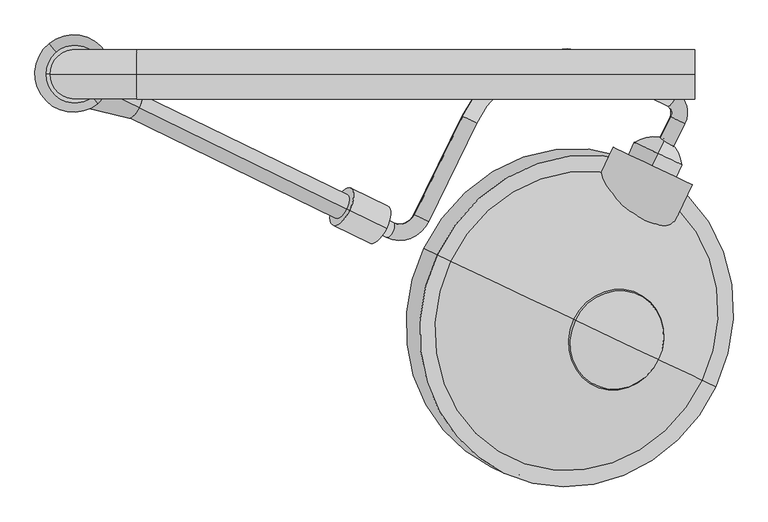
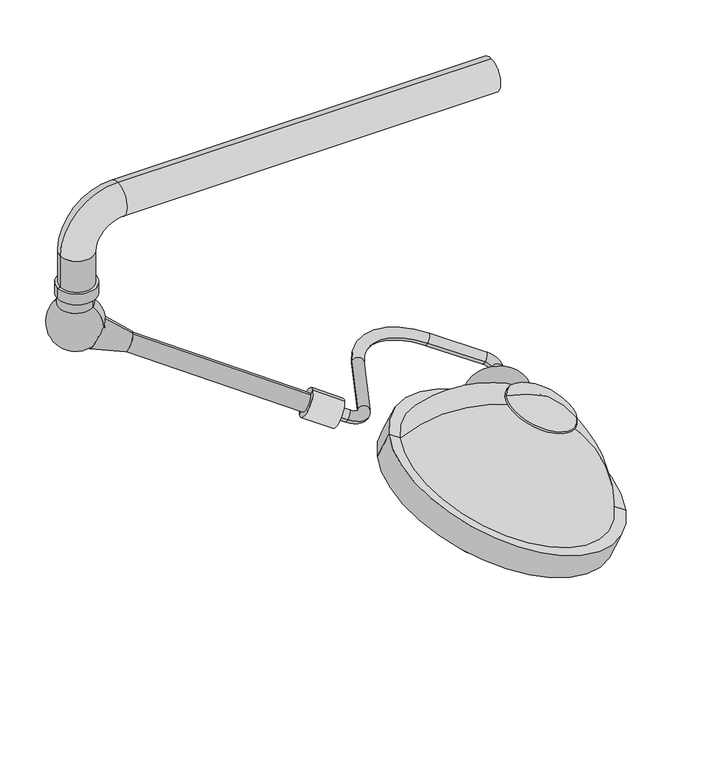
"""IFC4 building model written with IfcOpenShell, lengths in millimetres: proxy geometry, M7490 - Light, Surg, Ceiling Mtd, Dual, Unequal Dia Heads : M7490 - Light, Surg, Ceiling Mtd, Dual, Unequal Dia Heads."""

import ifcopenshell
import ifcopenshell.guid

model = None  # the IFC model being written
_history = None  # IfcOwnerHistory: only IFC2X3 demands one
_inside = {}  # id of a spatial element -> (the spatial element, [elements in it])
_under = {}  # id of a project, library or spatial element -> (it, [spatial elements below it])
_declared = {}  # id of a project -> (the project, [libraries it declares])
_typed = {}  # id of a type object -> (the type object, [elements of that type])
_made_of = {}  # id of a material, layer set ... -> (it, [elements and type objects made of it])


def new_model(schema):
    """Start an empty IFC model of exactly this schema.

    Asked for "IFC4X3", IfcOpenShell would pick the latest addendum, in which some entities
    have other attributes; the version numbers below select the first issue.
    IFC2X3 requires an IfcOwnerHistory on every rooted entity: one is made here for all.
    """
    global model, _history
    if schema == "IFC4X3":
        model = ifcopenshell.file(schema_version=(4, 3, 0, 0))
    else:
        model = ifcopenshell.file(schema=schema)
    _inside.clear()
    _under.clear()
    _declared.clear()
    _typed.clear()
    _made_of.clear()
    _history = None
    if model.schema == "IFC2X3":
        org = make("IfcOrganization", Name="unknown")
        user = make(
            "IfcPersonAndOrganization",
            ThePerson=make("IfcPerson", FamilyName="unknown"),
            TheOrganization=org,
        )
        app = make(
            "IfcApplication",
            ApplicationDeveloper=org,
            Version="unknown",
            ApplicationFullName="unknown",
            ApplicationIdentifier="unknown",
        )
        _history = make(
            "IfcOwnerHistory",
            OwningUser=user,
            OwningApplication=app,
            ChangeAction="ADDED",
            CreationDate=0,
        )
    return model


def make(cls, **values):
    """One entity of the class cls with the attributes given. An attribute that is None is left unset."""
    return model.create_entity(
        cls, **{name: value for name, value in values.items() if value is not None}
    )


def rooted(cls, **values):
    """An entity with a GlobalId (a new one), such as an element, a storey or a relation."""
    return make(cls, GlobalId=ifcopenshell.guid.new(), OwnerHistory=_history, **values)


def si_unit(unit_type, name, prefix=None):
    """IfcSIUnit, for example si_unit("LENGTHUNIT", "METRE", prefix="MILLI")."""
    return make("IfcSIUnit", UnitType=unit_type, Prefix=prefix, Name=name)


def assignment(units):
    """IfcUnitAssignment: the units of a project."""
    return None if units is None else make("IfcUnitAssignment", Units=units)


def point(xyz):
    """IfcCartesianPoint."""
    return None if xyz is None else make("IfcCartesianPoint", Coordinates=xyz)


def direction(xyz):
    """IfcDirection."""
    return None if xyz is None else make("IfcDirection", DirectionRatios=xyz)


def frame(location, z_axis=None, x_axis=None):
    """IfcAxis2Placement3D, a coordinate frame: its origin and axes. An axis left out is left unset."""
    return make(
        "IfcAxis2Placement3D",
        Location=point(location),
        Axis=direction(z_axis),
        RefDirection=direction(x_axis),
    )


def frame_2d(location, x_axis=None):
    """IfcAxis2Placement2D, a coordinate frame in the plane: its origin and x axis."""
    return make(
        "IfcAxis2Placement2D", Location=point(location), RefDirection=direction(x_axis)
    )


def origin():
    """The frame at (0, 0, 0) with its axes left unset."""
    return frame((0.0, 0.0, 0.0))


def origin_2d():
    """The frame at (0, 0) in the plane with its x axis left unset."""
    return frame_2d((0.0, 0.0))


def place(relative_to, where):
    """IfcLocalPlacement: puts the frame where relative to a parent placement (None: the world)."""
    return make(
        "IfcLocalPlacement", PlacementRelTo=relative_to, RelativePlacement=where
    )


def context(
    kind, dimensions, precision=None, world=None, true_north=None, identifier=None
):
    """IfcGeometricRepresentationContext, for example the 3D "Model" context."""
    return make(
        "IfcGeometricRepresentationContext",
        ContextIdentifier=identifier,
        ContextType=kind,
        CoordinateSpaceDimension=dimensions,
        Precision=precision,
        WorldCoordinateSystem=world,
        TrueNorth=true_north,
    )


def project(units=None, contexts=None):
    """IfcProject with its units and contexts."""
    return rooted(
        "IfcProject",
        Name="project",
        RepresentationContexts=contexts,
        UnitsInContext=assignment(units),
    )


def spatial(cls, under=None, at=None, **own):
    """A site, building, storey or space (cls), placed at a placement, below another one or the project."""
    s = rooted(cls, ObjectPlacement=at, **own)
    if under is not None:
        _under.setdefault(under.id(), (under, []))[1].append(s)
    return s


def polyline(points):
    """IfcPolyline through the points."""
    return make("IfcPolyline", Points=[point(p) for p in points])


def circle_curve(where, radius):
    """IfcCircle in the frame where."""
    return make("IfcCircle", Position=where, Radius=radius)


def ellipse_curve(where, semi_axis1, semi_axis2):
    """IfcEllipse in the frame where."""
    return make(
        "IfcEllipse", Position=where, SemiAxis1=semi_axis1, SemiAxis2=semi_axis2
    )


def trimmed(basis, trim1, trim2, sense, master):
    """IfcTrimmedCurve: the piece of a basis curve between two trims."""
    return make(
        "IfcTrimmedCurve",
        BasisCurve=basis,
        Trim1=trim1,
        Trim2=trim2,
        SenseAgreement=sense,
        MasterRepresentation=master,
    )


def segment(curve, same_sense, transition):
    """IfcCompositeCurveSegment."""
    return make(
        "IfcCompositeCurveSegment",
        Transition=transition,
        SameSense=same_sense,
        ParentCurve=curve,
    )


def composite_curve(segments, self_intersect=None):
    """IfcCompositeCurve: segments joined end to end."""
    return make("IfcCompositeCurve", Segments=segments, SelfIntersect=self_intersect)


def outline(outer, holes=None, kind="AREA"):
    """IfcArbitraryClosedProfileDef: a profile drawn as a closed curve; with holes, ...WithVoids."""
    if holes is None:
        return make("IfcArbitraryClosedProfileDef", ProfileType=kind, OuterCurve=outer)
    return make(
        "IfcArbitraryProfileDefWithVoids",
        ProfileType=kind,
        OuterCurve=outer,
        InnerCurves=holes,
    )


def extrude(swept, where, along, depth):
    """IfcExtrudedAreaSolid: the profile swept, set in the frame where, extruded along a direction by depth."""
    return make(
        "IfcExtrudedAreaSolid",
        SweptArea=swept,
        Position=where,
        ExtrudedDirection=direction(along),
        Depth=depth,
    )


def shape(context_of_items, identifier, shape_type, items):
    """IfcShapeRepresentation: the items that make up one representation, for example the "Body"."""
    return make(
        "IfcShapeRepresentation",
        ContextOfItems=context_of_items,
        RepresentationIdentifier=identifier,
        RepresentationType=shape_type,
        Items=items,
    )


def source(mapping_origin, context_of_items, identifier, shape_type, items):
    """IfcRepresentationMap: a shape defined once, which mapped items show again and again."""
    return make(
        "IfcRepresentationMap",
        MappingOrigin=mapping_origin,
        MappedRepresentation=shape(context_of_items, identifier, shape_type, items),
    )


def transform(
    local_origin,
    x_axis=None,
    y_axis=None,
    z_axis=None,
    scale=None,
    scale2=None,
    scale3=None,
    uniform=True,
):
    """IfcCartesianTransformationOperator3D, or its non-uniform kind. x_axis, y_axis, z_axis: its Axis1, 2, 3."""
    if uniform:
        return make(
            "IfcCartesianTransformationOperator3D",
            Axis1=direction(x_axis),
            Axis2=direction(y_axis),
            LocalOrigin=point(local_origin),
            Scale=scale,
            Axis3=direction(z_axis),
        )
    return make(
        "IfcCartesianTransformationOperator3DnonUniform",
        Axis1=direction(x_axis),
        Axis2=direction(y_axis),
        LocalOrigin=point(local_origin),
        Scale=scale,
        Axis3=direction(z_axis),
        Scale2=scale2,
        Scale3=scale3,
    )


def mapped(mapping_source, mapping_target):
    """IfcMappedItem: shows the shape of a source again, moved by a transform."""
    return make(
        "IfcMappedItem", MappingSource=mapping_source, MappingTarget=mapping_target
    )


def made_of(thing, what):
    """Note that an element or type object is made of a material, layer set ...; save() writes the relation."""
    if what is not None:
        _made_of.setdefault(what.id(), (what, []))[1].append(thing)
    return thing


def element(
    cls,
    number,
    at=None,
    inside=None,
    cuts=None,
    type_object=None,
    material=None,
    context=None,
    identifier="Body",
    shape_type=None,
    held_by="IfcProductDefinitionShape",
    body=None,
    shapes=None,
    **own,
):
    """One element of the class cls, such as IfcWall. Its Tag is "e" and its number.

    at: its placement. inside: the storey or other place that contains it. cuts: it is an
    opening in that element (IfcRelVoidsElement). A single representation is given by context,
    identifier, shape_type and body (its items); several are given by shapes. held_by: the class
    of the entity that holds the representations. save() writes the other relations.
    """
    e = rooted(cls, Tag="e%d" % number, ObjectPlacement=at, **own)
    if body is not None:
        shapes = [shape(context, identifier, shape_type, body)]
    if shapes is not None:
        e.Representation = make(held_by, Representations=shapes)
    if inside is not None:
        _inside.setdefault(inside.id(), (inside, []))[1].append(e)
    if cuts is not None:
        rooted(
            "IfcRelVoidsElement", RelatingBuildingElement=cuts, RelatedOpeningElement=e
        )
    if type_object is not None:
        _typed.setdefault(type_object.id(), (type_object, []))[1].append(e)
    return made_of(e, material)


def aggregate(whole, parts):
    """IfcRelAggregates: a whole, such as a stair, and the parts it consists of."""
    return rooted("IfcRelAggregates", RelatingObject=whole, RelatedObjects=parts)


def save(model, path):
    """Write the relations noted so far, then the file.

    IfcRelAggregates (storeys below a building ...), IfcRelContainedInSpatialStructure (elements
    in a storey), IfcRelDefinesByType, IfcRelAssociatesMaterial and IfcRelDeclares: one each for
    every whole, place, type object, material and project.
    """
    for whole, parts in _under.values():
        aggregate(whole, parts)
    for where, things in _inside.values():
        rooted(
            "IfcRelContainedInSpatialStructure",
            RelatedElements=things,
            RelatingStructure=where,
        )
    for kind, things in _typed.values():
        rooted("IfcRelDefinesByType", RelatedObjects=things, RelatingType=kind)
    for what, things in _made_of.values():
        rooted("IfcRelAssociatesMaterial", RelatedObjects=things, RelatingMaterial=what)
    for by, libraries in _declared.values():
        rooted("IfcRelDeclares", RelatingContext=by, RelatedDefinitions=libraries)
    model.write(path)


def plane_surface(at):
    """IfcPlane: the flat surface through the origin of the frame at, square to its z axis."""
    return make("IfcPlane", Position=at)


def cylinder_surface(at, radius):
    """IfcCylindricalSurface: all points at the distance radius from the z axis of the frame at."""
    return make("IfcCylindricalSurface", Position=at, Radius=radius)


def revolved_surface(curve, axis_point, axis_direction):
    """IfcSurfaceOfRevolution: the curve turned about the line through axis_point along axis_direction."""
    return make(
        "IfcSurfaceOfRevolution",
        SweptCurve=make("IfcArbitraryOpenProfileDef", ProfileType="CURVE", Curve=curve),
        AxisPosition=make("IfcAxis1Placement", Location=point(axis_point), Axis=direction(axis_direction)),
    )


def advanced_brep(points, edges, surfaces, faces):
    """IfcAdvancedBrep: a solid bounded by faces that lie on surfaces and meet in shared edges.

    An edge is (start, end): straight between two places in points (the first is 0);
    or (start, end, curve); or (start, end, curve, False) where it runs against its curve.
    A face is (place in surfaces, loops), or (place, loops, False) where it looks against
    its surface's normal. A loop lists edges by number (the first is 1), with a minus sign
    where the edge is run from its end to its start. The first loop is the outer one.
    """
    corners = [point(p) for p in points]
    vertices = [make("IfcVertexPoint", VertexGeometry=c) for c in corners]
    made = []
    for start, end, *more in edges:
        made.append(
            make(
                "IfcEdgeCurve",
                EdgeStart=vertices[start],
                EdgeEnd=vertices[end],
                EdgeGeometry=more[0] if more else make("IfcPolyline", Points=[corners[start], corners[end]]),
                SameSense=more[1] if len(more) > 1 else True,
            )
        )
    hull = []
    for where, loops, *sense in faces:
        bounds = []
        for j, loop in enumerate(loops):
            ring = [make("IfcOrientedEdge", EdgeElement=made[abs(k) - 1], Orientation=k > 0) for k in loop]
            bounds.append(
                make(
                    "IfcFaceOuterBound" if j == 0 else "IfcFaceBound",
                    Bound=make("IfcEdgeLoop", EdgeList=ring),
                    Orientation=True,
                )
            )
        hull.append(make("IfcAdvancedFace", Bounds=bounds, FaceSurface=surfaces[where], SameSense=sense[0] if sense else True))
    return make("IfcAdvancedBrep", Outer=make("IfcClosedShell", CfsFaces=hull))


def specialty_equipment_e6020135(model_context):
    return source(origin(), model_context, "Body", "SolidModel", [
        advanced_brep(
        [(-51.3241797, 670.2413617, 1699.7604265), (-72.1798458, 680.4133498, 1710.0915373), (-30.6483179, 712.6331606, 1699.7604265), (-51.503984, 722.8051486, 1710.0915373), (-56.3645035, 739.305827, 1715.2570926), (-45.2298764, 762.1351958, 1715.2570926), (-148.7448243, 812.6228093, 1766.5344952), (-159.8794514, 789.7934405, 1766.5344952), (-351.8212111, 713.8491561, 1828.5211596), (-372.6768772, 724.0211441, 1838.8522704), (-446.9378356, 571.7636159, 1838.8522704), (-426.0821694, 561.5916279, 1828.5211596), (-490.062756, 536.2768664, 1849.1833811), (-478.9281288, 559.1062352, 1849.1833811), (-557.8921303, 597.619552, 1888.2991704), (-569.0267574, 574.7901832, 1888.2991704)],
        [
            (0, 1, circle_curve(frame((-61.7520127, 675.3273558, 1704.9259819), z_axis=(-0.43837114678908723, -0.8987940462991623, 0.0), x_axis=(-0.8210892183528129, 0.40047196991074896, 0.4067366430758003)), 12.7)),
            (1, 0, circle_curve(frame((-61.7520127, 675.3273558, 1704.9259819), z_axis=(-0.43837114678908723, -0.8987940462991623, 0.0), x_axis=(-0.8210892183528129, 0.40047196991074896, 0.4067366430758003)), 12.7)),
            (0, 2),
            (2, 3, circle_curve(frame((-41.0761509, 717.7191546, 1704.9259819), z_axis=(-0.43837114678908723, -0.8987940462991623, 0.0), x_axis=(-0.8210892183528129, 0.40047196991074896, 0.4067366430758003)), 12.7)),
            (3, 1),
            (3, 2, circle_curve(frame((-41.0761509, 717.7191546, 1704.9259819), z_axis=(-0.43837114678908723, -0.8987940462991623, 0.0), x_axis=(-0.8210892183528129, 0.40047196991074896, 0.4067366430758003)), 12.7)),
            (4, 3, circle_curve(frame((-61.9318171, 727.8911427, 1715.2570926), z_axis=(-0.36557247320823727, 0.17830160866628114, -0.9135454576426009), x_axis=(0.8210892183528128, -0.400471969910749, -0.4067366430758004)), 12.7)),
            (2, 5, circle_curve(frame((-61.9318171, 727.8911427, 1715.2570926), z_axis=(0.36557247320823727, -0.17830160866628114, 0.9135454576426009), x_axis=(0.8210892183528128, -0.400471969910749, -0.4067366430758004)), 38.1)),
            (5, 4, circle_curve(frame((-50.79719, 750.7205114, 1715.2570926), z_axis=(0.8210892183528112, -0.4004719699107522, -0.4067366430758003), x_axis=(-0.4383711467890902, -0.8987940462991607, 0.0)), 12.7)),
            (4, 5, circle_curve(frame((-50.79719, 750.7205114, 1715.2570926), z_axis=(0.8210892183528081, -0.40047196991075856, -0.4067366430758003), x_axis=(-0.43837114678909606, -0.8987940462991579, 0.0)), 12.7)),
            (5, 6),
            (6, 7, circle_curve(frame((-154.3121378, 801.2081249, 1766.5344952), z_axis=(0.821089218352813, -0.40047196991074857, -0.40673664307580043), x_axis=(-0.4383711467890869, -0.8987940462991624, 0.0)), 12.7)),
            (7, 4),
            (7, 6, circle_curve(frame((-154.3121378, 801.2081249, 1766.5344952), z_axis=(0.821089218352813, -0.40047196991074857, -0.40673664307580043), x_axis=(-0.4383711467890869, -0.8987940462991624, 0.0)), 12.7)),
            (8, 7, circle_curve(frame((-226.6872142, 652.8172279, 1766.5344952), z_axis=(-0.36557247320823727, 0.17830160866628114, -0.9135454576426009), x_axis=(0.43837114678909317, 0.8987940462991594, 0.0)), 152.4)),
            (6, 9, circle_curve(frame((-226.6872142, 652.8172279, 1766.5344952), z_axis=(0.36557247320823727, -0.17830160866628114, 0.9135454576426009), x_axis=(0.43837114678909317, 0.8987940462991594, 0.0)), 177.8)),
            (9, 8, circle_curve(frame((-362.2490441, 718.9351501, 1833.686715), z_axis=(0.4383711467890851, 0.8987940462991633, 0.0), x_axis=(0.821089218352814, -0.40047196991074674, -0.40673664307580043)), 12.7)),
            (8, 9, circle_curve(frame((-362.2490441, 718.9351501, 1833.686715), z_axis=(0.4383711467890848, 0.8987940462991635, 0.0), x_axis=(0.8210892183528142, -0.4004719699107463, -0.40673664307580043)), 12.7)),
            (9, 10),
            (10, 11, circle_curve(frame((-436.5100025, 566.6776219, 1833.686715), z_axis=(0.43837114678908545, 0.898794046299163, 0.0), x_axis=(0.8210892183528139, -0.400471969910747, -0.4067366430758005)), 12.7)),
            (11, 8),
            (11, 10, circle_curve(frame((-436.5100025, 566.6776219, 1833.686715), z_axis=(0.43837114678908545, 0.898794046299163, 0.0), x_axis=(0.8210892183528139, -0.400471969910747, -0.4067366430758005)), 12.7)),
            (12, 11, circle_curve(frame((-467.7935017, 581.935604, 1849.1833811), z_axis=(0.36557247320823727, -0.17830160866628114, 0.9135454576426009), x_axis=(0.8210892183528169, -0.4004719699107408, -0.4067366430758004)), 50.8)),
            (10, 13, circle_curve(frame((-467.7935017, 581.935604, 1849.1833811), z_axis=(-0.36557247320823727, 0.17830160866628114, -0.9135454576426009), x_axis=(0.8210892183528169, -0.4004719699107408, -0.4067366430758004)), 25.4)),
            (13, 12, circle_curve(frame((-484.4954424, 547.6915508, 1849.1833811), z_axis=(0.8210892183528147, -0.40047196991074524, -0.4067366430758004), x_axis=(-0.4383711467890839, -0.8987940462991639, 0.0)), 12.7)),
            (12, 13, circle_curve(frame((-484.4954424, 547.6915508, 1849.1833811), z_axis=(0.8210892183528171, -0.40047196991074047, -0.4067366430758004), x_axis=(-0.4383711467890795, -0.898794046299166, 0.0)), 12.7)),
            (14, 15, circle_curve(frame((-563.4594439, 586.2048676, 1888.2991704), z_axis=(-0.821089218352815, 0.40047196991074563, 0.4067366430757997), x_axis=(-0.438371146789084, -0.8987940462991637, 0.0)), 12.7)),
            (15, 14, circle_curve(frame((-563.4594439, 586.2048676, 1888.2991704), z_axis=(-0.821089218352815, 0.40047196991074563, 0.4067366430757997), x_axis=(-0.438371146789084, -0.8987940462991637, 0.0)), 12.7)),
            (13, 14),
            (15, 12),
        ],
        [
            plane_surface(frame((-671.2712366, 972.6097446, 181.7710423), z_axis=(-0.43837114678908734, -0.8987940462991622, 0.0), x_axis=(0.3655724732082375, -0.17830160866628114, 0.9135454576426008))),
            cylinder_surface(frame((-61.7520127, 675.3273558, 1704.9259819), z_axis=(-0.43837114678908723, -0.8987940462991623, 0.0), x_axis=(-0.8210892183528129, 0.40047196991074896, 0.4067366430758003)), 12.7),
            revolved_surface(trimmed(ellipse_curve(frame((-41.0761509, 717.7191546, 1704.9259819), z_axis=(-0.43837114678908723, -0.8987940462991622, 0.0), x_axis=(-0.8210892183528128, 0.4004719699107489, 0.40673664307580043)), 12.7, 12.7), [point((-30.6483179, 712.6331606, 1699.7604265))], [point((-51.503984, 722.8051486, 1710.0915373))], True, "CARTESIAN"), (-671.451041, 1025.1735315, 192.1021531), (0.36557247320823727, -0.17830160866628114, 0.9135454576426009)),
            revolved_surface(trimmed(ellipse_curve(frame((-41.0761509, 717.7191546, 1704.9259819), z_axis=(-0.43837114678908723, -0.8987940462991622, 0.0), x_axis=(-0.8210892183528128, 0.4004719699107489, 0.40673664307580043)), 12.7, 12.7), [point((-51.503984, 722.8051486, 1710.0915373))], [point((-30.6483179, 712.6331606, 1699.7604265))], True, "CARTESIAN"), (-671.451041, 1025.1735315, 192.1021531), (0.36557247320823727, -0.17830160866628114, 0.9135454576426009)),
            cylinder_surface(frame((-50.79719, 750.7205114, 1715.2570926), z_axis=(0.821089218352813, -0.40047196991074857, -0.40673664307580043), x_axis=(-0.4383711467890869, -0.8987940462991624, 0.0)), 12.7),
            revolved_surface(trimmed(ellipse_curve(frame((-154.3121378, 801.2081249, 1766.5344952), z_axis=(0.8210892183528098, -0.40047196991075545, -0.4067366430758005), x_axis=(-0.4383711467890932, -0.8987940462991594, 0.0)), 12.7, 12.7), [point((-148.7448243, 812.6228093, 1766.5344952))], [point((-159.8794514, 789.7934405, 1766.5344952))], True, "CARTESIAN"), (-836.2064381, 950.0996167, 243.3795556), (0.36557247320823727, -0.17830160866628114, 0.9135454576426009)),
            revolved_surface(trimmed(ellipse_curve(frame((-154.3121378, 801.2081249, 1766.5344952), z_axis=(0.8210892183528098, -0.40047196991075545, -0.4067366430758005), x_axis=(-0.4383711467890932, -0.8987940462991594, 0.0)), 12.7, 12.7), [point((-159.8794514, 789.7934405, 1766.5344952))], [point((-148.7448243, 812.6228093, 1766.5344952))], True, "CARTESIAN"), (-836.2064381, 950.0996167, 243.3795556), (0.36557247320823727, -0.17830160866628114, 0.9135454576426009)),
            cylinder_surface(frame((-362.2490441, 718.9351501, 1833.686715), z_axis=(0.43837114678908556, 0.8987940462991633, 0.0), x_axis=(0.8210892183528139, -0.400471969910747, -0.4067366430758005)), 12.7),
            revolved_surface(trimmed(ellipse_curve(frame((-436.5100025, 566.6776219, 1833.686715), z_axis=(0.43837114678907957, 0.898794046299166, 0.0), x_axis=(0.821089218352817, -0.4004719699107405, -0.40673664307580043)), 12.7, 12.7), [point((-446.9378356, 571.7636159, 1838.8522704))], [point((-426.0821694, 561.5916279, 1828.5211596))], True, "CARTESIAN"), (-1077.3127256, 879.2179928, 326.0284415), (-0.36557247320823727, 0.17830160866628114, -0.9135454576426009)),
            revolved_surface(trimmed(ellipse_curve(frame((-436.5100025, 566.6776219, 1833.686715), z_axis=(0.43837114678907957, 0.898794046299166, 0.0), x_axis=(0.821089218352817, -0.4004719699107405, -0.40673664307580043)), 12.7, 12.7), [point((-426.0821694, 561.5916279, 1828.5211596))], [point((-446.9378356, 571.7636159, 1838.8522704))], True, "CARTESIAN"), (-1077.3127256, 879.2179928, 326.0284415), (-0.36557247320823727, 0.17830160866628114, -0.9135454576426009)),
            plane_surface(frame((-1172.9786678, 883.4872565, 365.1442308), z_axis=(-0.821089218352815, 0.40047196991074574, 0.4067366430757996), x_axis=(0.3655724732082366, -0.1783016086662806, 0.9135454576426013))),
            cylinder_surface(frame((-484.4954424, 547.6915508, 1849.1833811), z_axis=(0.8210892183528148, -0.4004719699107455, -0.4067366430757996), x_axis=(-0.438371146789084, -0.8987940462991637, 0.0)), 12.7),
        ],
        [
            (0, [[1, 2]]),
            (1, [[-1, 3, 4, 5]]),
            (1, [[-2, -5, 6, -3]]),
            (2, [[7, -4, 8, 9]]),
            (3, [[-8, -6, -7, 10]]),
            (4, [[-9, 11, 12, 13]]),
            (4, [[-10, -13, 14, -11]]),
            (5, [[15, -12, 16, 17]]),
            (6, [[-16, -14, -15, 18]]),
            (7, [[-17, 19, 20, 21]]),
            (7, [[-18, -21, 22, -19]]),
            (8, [[23, -20, 24, 25]]),
            (9, [[-24, -22, -23, 26]]),
            (10, [[27, 28]]),
            (11, [[-25, 29, -28, 30]]),
            (11, [[-26, -30, -27, -29]]),
        ],
    ),
        advanced_brep(
        [(-70.9853036, 666.0888501, 1662.093259), (-70.9853036, 666.0888501, 1743.3108067), (-79.9012214, 647.2586456, 1743.3108067), (-79.9012214, 647.2586456, 1662.093259), (-59.9841849, 689.3229491, 1702.7020328), (-79.9012214, 647.2586456, 1702.7020328)],
        [
            (0, 1, circle_curve(frame((-70.9853036, 666.0888501, 1702.7020328), z_axis=(-0.4279431442574036, -0.9038056568107367, 0.0), x_axis=(0.0, 0.0, 1.0)), 40.6087738)),
            (1, 2),
            (2, 3, circle_curve(frame((-79.9012214, 647.2586456, 1702.7020328), z_axis=(0.4279431442574036, 0.9038056568107367, 0.0), x_axis=(0.0, 0.0, 1.0)), 40.6087738)),
            (3, 0),
            (1, 0, circle_curve(frame((-70.9853036, 666.0888501, 1702.7020328), z_axis=(-0.4279431442574036, -0.9038056568107367, 0.0), x_axis=(0.0, 0.0, 1.0)), 40.6087738)),
            (3, 2, circle_curve(frame((-79.9012214, 647.2586456, 1702.7020328), z_axis=(0.4279431442574036, 0.9038056568107367, 0.0), x_axis=(0.0, 0.0, 1.0)), 40.6087738)),
            (4, 1, circle_curve(frame((-83.4268503, 639.8126019, 1696.4653606), z_axis=(0.9038056568107367, -0.42794314425740376, 0.0), x_axis=(-0.42794314425740393, -0.9038056568107365, 0.0)), 55.1337385)),
            (0, 4, circle_curve(frame((-83.4268503, 639.8126019, 1708.9387051), z_axis=(0.9038056568107369, -0.4279431442574031, 0.0), x_axis=(-0.42794314425740326, -0.9038056568107368, 0.0)), 55.1337385)),
            (2, 5),
            (5, 3),
        ],
        [
            cylinder_surface(frame((-79.9012214, 647.2586456, 1702.7020328), z_axis=(0.4279431442574036, 0.9038056568107367, 0.0), x_axis=(0.0, 0.0, 1.0)), 40.6087738),
            revolved_surface(trimmed(ellipse_curve(frame((-83.4268503, 639.8126019, 1696.4653606), z_axis=(-0.9038056568107367, 0.42794314425740376, 0.0), x_axis=(-0.42794314425740393, -0.9038056568107365, 0.0)), 55.1337385, 55.1337385), [point((-70.9853036, 666.0888501, 1743.3108067))], [point((-59.9841849, 689.3229491, 1702.7020328))], True, "CARTESIAN"), (-79.9012214, 647.2586456, 1702.7020328), (0.4279431442574036, 0.9038056568107367, 0.0)),
            revolved_surface(trimmed(ellipse_curve(frame((-83.4268503, 639.8126019, 1696.4653606), z_axis=(-0.9038056568107365, 0.42794314425740393, 0.0), x_axis=(-0.4279431442574041, -0.9038056568107364, 0.0)), 55.1337385, 55.1337385), [point((-70.9853036, 666.0888501, 1743.3108067))], [point((-59.9841849, 689.3229491, 1702.7020328))], True, "CARTESIAN"), (-79.9012214, 647.2586456, 1702.7020328), (0.4279431442574036, 0.9038056568107367, 0.0)),
            plane_surface(frame((-79.9012214, 647.2586456, 1702.7020328), z_axis=(-0.42794314425740343, -0.9038056568107368, 0.0), x_axis=(0.0, 0.0, 1.0))),
        ],
        [
            (0, [[1, 2, 3, 4]]),
            (0, [[5, -4, 6, -2]]),
            (1, [[7, -1, 8]]),
            (2, [[-8, -5, -7]]),
            (3, [[-3, 9, 10]]),
            (3, [[-6, -10, -9]]),
        ],
    ),
        advanced_brep(
        [(-198.2891405, 408.2286063, 1882.6946884), (-70.3964825, 347.6726828, 1819.6927814), (-123.8504881, 372.982632, 1877.268084), (-200.9060117, 409.4676693, 1880.0876662), (-70.3964825, 347.6726828, 1815.7966478), (-129.8474904, 375.822154, 1862.3650044)],
        [
            (0, 1, circle_curve(frame((-134.3428115, 377.9506446, 1851.1937349), z_axis=(0.3676108788441171, -0.17406015792255894, 0.9135454576426013), x_axis=(0.8256675523711364, -0.3909455155656434, -0.4067366430757995)), 77.4480344)),
            (1, 2, circle_curve(frame((-222.0261973, 419.4678707, 1706.5205002), z_axis=(-0.42794314425740376, -0.9038056568107369, 0.0), x_axis=(-0.9038056568107369, 0.4279431442574038, 0.0)), 202.3711557)),
            (2, 0, circle_curve(frame((-172.8421817, 396.1797201, 1682.2916913), z_axis=(-0.427943144257401, -0.9038056568107382, 0.0), x_axis=(0.604764027172337, -0.2863498556040709, -0.7431448254773931)), 202.3711557)),
            (1, 0, circle_curve(frame((-134.3428115, 377.9506446, 1851.1937349), z_axis=(0.3676108788441171, -0.17406015792255894, 0.9135454576426013), x_axis=(0.8256675523711364, -0.3909455155656434, -0.4067366430757995)), 77.4480344)),
            (3, 4, circle_curve(frame((-135.6512471, 378.5701761, 1847.942157), z_axis=(0.3676108788441171, -0.17406015792255894, 0.9135454576426013), x_axis=(0.8256675523711364, -0.3909455155656434, -0.4067366430757995)), 79.0327347)),
            (4, 1),
            (0, 3),
            (4, 3, circle_curve(frame((-135.6512471, 378.5701761, 1847.942157), z_axis=(0.3676108788441171, -0.17406015792255894, 0.9135454576426013), x_axis=(0.8256675523711364, -0.3909455155656434, -0.4067366430757995)), 79.0327347)),
            (5, 4, circle_curve(frame((-246.9439851, 431.2661997, 1609.6195886), z_axis=(0.42794314425740376, 0.9038056568107369, 0.0), x_axis=(-0.9038056568107369, 0.4279431442574038, 0.0)), 284.0173877)),
            (3, 5, circle_curve(frame((-221.2532479, 419.1018867, 1596.9639329), z_axis=(0.427943144257401, 0.9038056568107382, 0.0), x_axis=(0.604764027172337, -0.2863498556040709, -0.7431448254773931)), 284.0173877)),
        ],
        [
            revolved_surface(trimmed(ellipse_curve(frame((-222.0261973, 419.4678707, 1706.5205002), z_axis=(0.42794314425740376, 0.9038056568107369, 0.0), x_axis=(-0.9038056568107369, 0.4279431442574038, 0.0)), 202.3711557, 202.3711557), [point((-123.8504881, 372.982632, 1877.268084))], [point((-70.3964825, 347.6726828, 1819.6927814))], True, "CARTESIAN"), (-169.8512246, 394.7635311, 1762.9521965), (-0.3676108788441171, 0.17406015792255894, -0.9135454576426013)),
            revolved_surface(trimmed(ellipse_curve(frame((-222.0261973, 419.4678707, 1706.5205002), z_axis=(0.42794314425740376, 0.9038056568107369, 0.0), x_axis=(-0.9038056568107369, 0.42794314425740376, 0.0)), 202.3711557, 202.3711557), [point((-123.8504881, 372.982632, 1877.268084))], [point((-70.3964825, 347.6726828, 1819.6927814))], True, "CARTESIAN"), (-169.8512246, 394.7635311, 1762.9521965), (-0.3676108788441171, 0.17406015792255894, -0.9135454576426013)),
            revolved_surface(polyline([(-70.3964825, 347.6726828, 1819.6927814), (-70.3964825, 347.6726828, 1815.7966478)]), (-169.8512246, 394.7635311, 1762.9521965), (-0.3676108788441171, 0.17406015792255894, -0.9135454576426013)),
            revolved_surface(trimmed(ellipse_curve(frame((-246.9439851, 431.2661997, 1609.6195886), z_axis=(-0.42794314425740376, -0.9038056568107369, 0.0), x_axis=(-0.9038056568107369, 0.4279431442574038, 0.0)), 284.0173877, 284.0173877), [point((-70.3964825, 347.6726828, 1815.7966478))], [point((-129.8474904, 375.822154, 1862.3650044))], True, "CARTESIAN"), (-169.8512246, 394.7635311, 1762.9521965), (-0.3676108788441171, 0.17406015792255894, -0.9135454576426013)),
            revolved_surface(trimmed(ellipse_curve(frame((-246.9439851, 431.2661997, 1609.6195886), z_axis=(-0.42794314425740376, -0.9038056568107369, 0.0), x_axis=(-0.9038056568107369, 0.42794314425740376, 0.0)), 284.0173877, 284.0173877), [point((-70.3964825, 347.6726828, 1815.7966478))], [point((-129.8474904, 375.822154, 1862.3650044))], True, "CARTESIAN"), (-169.8512246, 394.7635311, 1762.9521965), (-0.3676108788441171, 0.17406015792255894, -0.9135454576426013)),
        ],
        [
            (0, [[1, 2, 3]]),
            (1, [[4, -3, -2]]),
            (2, [[5, 6, -1, 7]]),
            (2, [[8, -7, -4, -6]]),
            (3, [[9, -5, 10]]),
            (4, [[-10, -8, -9]]),
        ],
    ),
        advanced_brep(
        [(-266.4821549, 440.5173321, 1522.8158117), (-276.9681328, 445.4823401, 1527.9813671), (-255.996177, 435.552324, 1517.6502563), (-263.0629437, 438.898369, 1507.6425198), (-278.9613242, 446.4260968, 1515.4743086), (-271.0121339, 442.6622329, 1511.5584142)],
        [
            (0, 1),
            (1, 2, circle_curve(frame((-266.4821549, 440.5173321, 1522.8158117), z_axis=(0.36761087884411703, -0.17406015792255897, 0.9135454576426013), x_axis=(-0.8256675523711364, 0.3909455155656434, 0.40673664307579943)), 12.7)),
            (2, 0),
            (2, 1, circle_curve(frame((-266.4821549, 440.5173321, 1522.8158117), z_axis=(0.36761087884411703, -0.17406015792255897, 0.9135454576426013), x_axis=(-0.8256675523711364, 0.3909455155656434, 0.40673664307579943)), 12.7)),
            (3, 4, circle_curve(frame((-271.0121339, 442.6622329, 1511.5584142), z_axis=(-0.36761087884411703, 0.17406015792255897, -0.9135454576426013), x_axis=(-0.8256675523711364, 0.3909455155656434, 0.40673664307579943)), 9.6275919)),
            (4, 5),
            (5, 3),
            (4, 3, circle_curve(frame((-271.0121339, 442.6622329, 1511.5584142), z_axis=(-0.36761087884411703, 0.17406015792255897, -0.9135454576426013), x_axis=(-0.8256675523711364, 0.3909455155656434, 0.40673664307579943)), 9.6275919)),
            (1, 4),
            (3, 2),
        ],
        [
            plane_surface(frame((-266.4821549, 440.5173321, 1522.8158117), z_axis=(0.36761087884411714, -0.1740601579225589, 0.9135454576426014), x_axis=(-0.8256675523711364, 0.3909455155656434, 0.40673664307579943))),
            plane_surface(frame((-271.0121339, 442.6622329, 1511.5584142), z_axis=(-0.36761087884411714, 0.1740601579225589, -0.9135454576426014), x_axis=(-0.8256675523711364, 0.3909455155656434, 0.40673664307579943))),
            revolved_surface(polyline([(-278.9613242, 446.4260968, 1515.4743086), (-276.9681328, 445.4823401, 1527.9813671)]), (-229.1328896, 422.83282, 1615.6320302), (0.36761087884411703, -0.17406015792255897, 0.9135454576426013)),
        ],
        [
            (0, [[1, 2, 3]]),
            (0, [[-3, 4, -1]]),
            (1, [[5, 6, 7]]),
            (1, [[8, -7, -6]]),
            (2, [[-2, 9, -5, 10]]),
            (2, [[-4, -10, -8, -9]]),
        ],
    ),
        advanced_brep(
        [(-229.1328896, 422.83282, 1615.6320302), (-244.8618565, 430.2803321, 1623.3803632), (-213.4039227, 415.385308, 1607.8836971), (-250.753188, 433.06982, 1515.0674786), (-282.2111217, 447.9648442, 1530.5641447), (-266.4821549, 440.5173321, 1522.8158117)],
        [
            (0, 1),
            (1, 2, circle_curve(frame((-229.1328896, 422.83282, 1615.6320302), z_axis=(0.36761087884411703, -0.17406015792255897, 0.9135454576426013), x_axis=(-0.8256675523711364, 0.3909455155656434, 0.40673664307579943)), 19.05)),
            (2, 0),
            (2, 1, circle_curve(frame((-229.1328896, 422.83282, 1615.6320302), z_axis=(0.36761087884411703, -0.17406015792255897, 0.9135454576426013), x_axis=(-0.8256675523711364, 0.3909455155656434, 0.40673664307579943)), 19.05)),
            (3, 4, circle_curve(frame((-266.4821549, 440.5173321, 1522.8158117), z_axis=(-0.36761087884411703, 0.17406015792255897, -0.9135454576426013), x_axis=(-0.8256675523711364, 0.3909455155656434, 0.40673664307579943)), 19.05)),
            (4, 5),
            (5, 3),
            (4, 3, circle_curve(frame((-266.4821549, 440.5173321, 1522.8158117), z_axis=(-0.36761087884411703, 0.17406015792255897, -0.9135454576426013), x_axis=(-0.8256675523711364, 0.3909455155656434, 0.40673664307579943)), 19.05)),
            (1, 4),
            (3, 2),
        ],
        [
            plane_surface(frame((-229.1328896, 422.83282, 1615.6320302), z_axis=(0.36761087884411714, -0.1740601579225589, 0.9135454576426014), x_axis=(-0.8256675523711364, 0.3909455155656434, 0.40673664307579943))),
            plane_surface(frame((-266.4821549, 440.5173321, 1522.8158117), z_axis=(-0.36761087884411714, 0.1740601579225589, -0.9135454576426014), x_axis=(-0.8256675523711364, 0.3909455155656434, 0.40673664307579943))),
            cylinder_surface(frame((-229.1328896, 422.83282, 1615.6320302), z_axis=(0.36761087884411703, -0.17406015792255897, 0.9135454576426013), x_axis=(-0.8256675523711364, 0.3909455155656434, 0.40673664307579943)), 19.05),
        ],
        [
            (0, [[1, 2, 3]]),
            (0, [[-3, 4, -1]]),
            (1, [[5, 6, 7]]),
            (1, [[8, -7, -6]]),
            (2, [[-2, 9, -5, 10]]),
            (2, [[-4, -10, -8, -9]]),
        ],
    ),
        advanced_brep(
        [(-222.1299023, 419.516974, 1633.0350712), (-258.830825, 436.8945022, 1651.1145149), (-185.4289796, 402.1394459, 1614.9556274), (-192.4319669, 405.4552919, 1597.5525864), (-265.8338123, 440.2103482, 1633.711474), (-229.1328896, 422.83282, 1615.6320302)],
        [
            (0, 1),
            (1, 2, circle_curve(frame((-222.1299023, 419.516974, 1633.0350712), z_axis=(0.3676108788441165, -0.1740601579225587, 0.9135454576426016), x_axis=(-0.8256675523711366, 0.3909455155656435, 0.4067366430757988)), 44.45)),
            (2, 0),
            (2, 1, circle_curve(frame((-222.1299023, 419.516974, 1633.0350712), z_axis=(0.3676108788441165, -0.1740601579225587, 0.9135454576426016), x_axis=(-0.8256675523711366, 0.3909455155656435, 0.4067366430757988)), 44.45)),
            (3, 4, circle_curve(frame((-229.1328896, 422.83282, 1615.6320302), z_axis=(-0.3676108788441165, 0.1740601579225587, -0.9135454576426016), x_axis=(-0.8256675523711366, 0.3909455155656435, 0.4067366430757988)), 44.45)),
            (4, 5),
            (5, 3),
            (4, 3, circle_curve(frame((-229.1328896, 422.83282, 1615.6320302), z_axis=(-0.3676108788441165, 0.1740601579225587, -0.9135454576426016), x_axis=(-0.8256675523711366, 0.3909455155656435, 0.4067366430757988)), 44.45)),
            (1, 4),
            (3, 2),
        ],
        [
            plane_surface(frame((-222.1299023, 419.516974, 1633.0350712), z_axis=(0.3676108788441166, -0.17406015792255863, 0.9135454576426016), x_axis=(-0.8256675523711366, 0.3909455155656435, 0.4067366430757988))),
            plane_surface(frame((-229.1328896, 422.83282, 1615.6320302), z_axis=(-0.3676108788441166, 0.17406015792255863, -0.9135454576426016), x_axis=(-0.8256675523711366, 0.3909455155656435, 0.4067366430757988))),
            cylinder_surface(frame((-222.1299023, 419.516974, 1633.0350712), z_axis=(0.3676108788441165, -0.1740601579225587, 0.9135454576426016), x_axis=(-0.8256675523711366, 0.3909455155656435, 0.4067366430757988)), 44.45),
        ],
        [
            (0, [[1, 2, 3]]),
            (0, [[-3, 4, -1]]),
            (1, [[5, 6, 7]]),
            (1, [[8, -7, -6]]),
            (2, [[-2, 9, -5, 10]]),
            (2, [[-4, -10, -8, -9]]),
        ],
    ),
        advanced_brep(
        [(-217.8648709, 417.4975233, 1643.6340505), (-265.0517715, 439.8400595, 1666.8790497), (-170.6779703, 395.1549871, 1620.3890514), (-179.2080332, 399.1938885, 1611.8910927), (-265.0517715, 439.8400595, 1654.1790497), (-222.1299023, 419.516974, 1633.0350712)],
        [
            (0, 1),
            (1, 2, circle_curve(frame((-217.8648709, 417.4975233, 1643.6340505), z_axis=(0.36761087884411725, -0.17406015792255908, 0.9135454576426012), x_axis=(-0.8256675523711363, 0.39094551556564333, 0.4067366430757997)), 57.15)),
            (2, 0),
            (2, 1, circle_curve(frame((-217.8648709, 417.4975233, 1643.6340505), z_axis=(0.36761087884411725, -0.17406015792255908, 0.9135454576426012), x_axis=(-0.8256675523711363, 0.39094551556564333, 0.4067366430757997)), 57.15)),
            (3, 4, circle_curve(frame((-222.1299023, 419.516974, 1633.0350712), z_axis=(-0.36761087884411725, 0.17406015792255908, -0.9135454576426012), x_axis=(-0.8256675523711363, 0.39094551556564333, 0.4067366430757997)), 51.9844446)),
            (4, 5),
            (5, 3),
            (4, 3, circle_curve(frame((-222.1299023, 419.516974, 1633.0350712), z_axis=(-0.36761087884411725, 0.17406015792255908, -0.9135454576426012), x_axis=(-0.8256675523711363, 0.39094551556564333, 0.4067366430757997)), 51.9844446)),
            (1, 4),
            (3, 2),
        ],
        [
            plane_surface(frame((-217.8648709, 417.4975233, 1643.6340505), z_axis=(0.36761087884411736, -0.17406015792255902, 0.9135454576426013), x_axis=(-0.8256675523711363, 0.39094551556564333, 0.4067366430757997))),
            plane_surface(frame((-222.1299023, 419.516974, 1633.0350712), z_axis=(-0.36761087884411736, 0.17406015792255902, -0.9135454576426013), x_axis=(-0.8256675523711363, 0.39094551556564333, 0.4067366430757997))),
            revolved_surface(polyline([(-265.0517715, 439.8400595, 1654.1790497), (-265.0517715, 439.8400595, 1666.8790497)]), (-217.8648709, 417.4975233, 1643.6340505), (0.36761087884411725, -0.17406015792255908, 0.9135454576426012)),
        ],
        [
            (0, [[1, 2, 3]]),
            (0, [[-3, 4, -1]]),
            (1, [[5, 6, 7]]),
            (1, [[8, -7, -6]]),
            (2, [[-2, 9, -5, 10]]),
            (2, [[-4, -10, -8, -9]]),
        ],
    ),
        extrude(outline(composite_curve([segment(polyline([(-25.1937137, -4.6953206), (31.6273953, -132.3176211)]), True, "CONTINUOUS"), segment(trimmed(circle_curve(frame_2d((0.0, -69.9387006)), 69.9387006), [point((31.6273953, -132.3176211))], [point((-25.1937137, -4.6953206))], False, "CARTESIAN"), True, "CONTINUOUS")], self_intersect=False)), frame((-180.69854, 601.7570747, 1699.0600142), z_axis=(0.42794314425740343, 0.9038056568107368, 0.0), x_axis=(0.0, 0.0, -1.0)), (0.0, 0.0, 1.0), 84.2600986),
        advanced_brep(
        [(-390.8465006, 499.4026342, 1791.4059477), (-2.8653177, 315.6973364, 1600.2803991), (-136.3788609, 378.9146941, 1846.1339726), (-385.1187358, 496.6905935, 1788.5843619), (-8.5930825, 318.4093771, 1603.1019849), (-138.6621528, 379.9958105, 1840.4597908)],
        [
            (0, 1, circle_curve(frame((-196.8559092, 407.5499853, 1695.8431734), z_axis=(0.3676108788441172, -0.17406015792255902, 0.9135454576426013), x_axis=(0.8256675523711364, -0.3909455155656434, -0.4067366430757996)), 234.95)),
            (1, 2, circle_curve(frame((-250.7671057, 433.0764099, 1602.7798508), z_axis=(-0.4279431442574038, -0.9038056568107369, 0.0), x_axis=(-0.9038056568107368, 0.4279431442574038, 0.0)), 274.297996)),
            (2, 0, circle_curve(frame((-223.289049, 420.0658186, 1589.2437338), z_axis=(-0.42794314425740104, -0.9038056568107381, 0.0), x_axis=(0.6047640271723369, -0.28634985560407084, -0.7431448254773931)), 274.297996)),
            (1, 0, circle_curve(frame((-196.8559092, 407.5499853, 1695.8431734), z_axis=(0.3676108788441172, -0.17406015792255902, 0.9135454576426013), x_axis=(0.8256675523711364, -0.3909455155656434, -0.4067366430757996)), 234.95)),
            (3, 4, circle_curve(frame((-196.8559092, 407.5499853, 1695.8431734), z_axis=(0.3676108788441172, -0.17406015792255902, 0.9135454576426013), x_axis=(0.8256675523711364, -0.3909455155656434, -0.4067366430757996)), 228.012868)),
            (4, 1),
            (0, 3),
            (4, 3, circle_curve(frame((-196.8559092, 407.5499853, 1695.8431734), z_axis=(0.3676108788441172, -0.17406015792255902, 0.9135454576426013), x_axis=(0.8256675523711364, -0.3909455155656434, -0.4067366430757996)), 228.012868)),
            (5, 4, circle_curve(frame((-250.6075587, 433.000866, 1603.0552661), z_axis=(0.4279431442574038, 0.9038056568107369, 0.0), x_axis=(-0.9038056568107368, 0.4279431442574038, 0.0)), 267.7726988)),
            (3, 5, circle_curve(frame((-223.2108217, 420.0287788, 1589.5592085), z_axis=(0.42794314425740104, 0.9038056568107381, 0.0), x_axis=(0.6047640271723369, -0.28634985560407084, -0.7431448254773931)), 267.7726988)),
        ],
        [
            revolved_surface(trimmed(ellipse_curve(frame((-250.7671057, 433.0764099, 1602.7798508), z_axis=(0.4279431442574038, 0.9038056568107369, 0.0), x_axis=(-0.9038056568107368, 0.4279431442574038, 0.0)), 274.297996, 274.297996), [point((-136.3788609, 378.9146941, 1846.1339726))], [point((-2.8653177, 315.6973364, 1600.2803991))], True, "CARTESIAN"), (-196.8559092, 407.5499853, 1695.8431734), (-0.3676108788441172, 0.17406015792255902, -0.9135454576426013)),
            revolved_surface(trimmed(ellipse_curve(frame((-250.7671057, 433.0764099, 1602.7798508), z_axis=(0.4279431442574037, 0.9038056568107367, 0.0), x_axis=(-0.9038056568107368, 0.42794314425740376, 0.0)), 274.297996, 274.297996), [point((-136.3788609, 378.9146941, 1846.1339726))], [point((-2.8653177, 315.6973364, 1600.2803991))], True, "CARTESIAN"), (-196.8559092, 407.5499853, 1695.8431734), (-0.3676108788441172, 0.17406015792255902, -0.9135454576426013)),
            plane_surface(frame((-196.8559092, 407.5499853, 1695.8431734), z_axis=(-0.3676108788441172, 0.17406015792255894, -0.9135454576426013), x_axis=(0.8256675523711363, -0.39094551556564333, -0.40673664307579954))),
            revolved_surface(trimmed(ellipse_curve(frame((-250.6075587, 433.000866, 1603.0552661), z_axis=(-0.4279431442574038, -0.9038056568107369, 0.0), x_axis=(-0.9038056568107368, 0.4279431442574038, 0.0)), 267.7726988, 267.7726988), [point((-8.5930825, 318.4093771, 1603.1019849))], [point((-138.6621528, 379.9958105, 1840.4597908))], True, "CARTESIAN"), (-196.8559092, 407.5499853, 1695.8431734), (-0.3676108788441172, 0.17406015792255902, -0.9135454576426013)),
            revolved_surface(trimmed(ellipse_curve(frame((-250.6075587, 433.000866, 1603.0552661), z_axis=(-0.4279431442574037, -0.9038056568107367, 0.0), x_axis=(-0.9038056568107368, 0.42794314425740376, 0.0)), 267.7726988, 267.7726988), [point((-8.5930825, 318.4093771, 1603.1019849))], [point((-138.6621528, 379.9958105, 1840.4597908))], True, "CARTESIAN"), (-196.8559092, 407.5499853, 1695.8431734), (-0.3676108788441172, 0.17406015792255902, -0.9135454576426013)),
        ],
        [
            (0, [[1, 2, 3]]),
            (1, [[4, -3, -2]]),
            (2, [[5, 6, -1, 7]]),
            (2, [[8, -7, -4, -6]]),
            (3, [[9, -5, 10]]),
            (4, [[-10, -8, -9]]),
        ],
    ),
        advanced_brep(
        [(-432.8274181, 519.2801883, 1749.5279355), (-2.9023236, 315.7148583, 1537.7401655), (18.1066381, 305.7673203, 1589.9492884), (-411.8184564, 509.3326503, 1801.7370584), (-427.5844292, 516.7976843, 1746.9451578), (-8.1453126, 318.1973624, 1540.3229432), (-408.9097965, 507.9554283, 1793.3532671), (10.5293201, 309.3551063, 1586.7310524), (-199.1902382, 408.6552673, 1690.0421598), (-196.8559092, 407.5499853, 1695.8431734)],
        [
            (0, 1, circle_curve(frame((-217.8648709, 417.4975233, 1643.6340505), z_axis=(0.3676108788441169, -0.17406015792255886, 0.9135454576426014), x_axis=(0.8256675523711365, -0.39094551556564344, -0.40673664307579926)), 260.35)),
            (1, 2),
            (2, 3, circle_curve(frame((-196.8559092, 407.5499853, 1695.8431734), z_axis=(-0.3676108788441169, 0.17406015792255886, -0.9135454576426014), x_axis=(0.8256675523711365, -0.39094551556564344, -0.40673664307579926)), 260.35)),
            (3, 0),
            (1, 0, circle_curve(frame((-217.8648709, 417.4975233, 1643.6340505), z_axis=(0.3676108788441169, -0.17406015792255886, 0.9135454576426014), x_axis=(0.8256675523711365, -0.39094551556564344, -0.40673664307579926)), 260.35)),
            (3, 2, circle_curve(frame((-196.8559092, 407.5499853, 1695.8431734), z_axis=(-0.3676108788441169, 0.17406015792255886, -0.9135454576426014), x_axis=(0.8256675523711365, -0.39094551556564344, -0.40673664307579926)), 260.35)),
            (4, 5, circle_curve(frame((-217.8648709, 417.4975233, 1643.6340505), z_axis=(0.3676108788441169, -0.17406015792255886, 0.9135454576426014), x_axis=(0.8256675523711365, -0.39094551556564344, -0.40673664307579926)), 254.0)),
            (5, 1),
            (0, 4),
            (5, 4, circle_curve(frame((-217.8648709, 417.4975233, 1643.6340505), z_axis=(0.3676108788441169, -0.17406015792255886, 0.9135454576426014), x_axis=(0.8256675523711365, -0.39094551556564344, -0.40673664307579926)), 254.0)),
            (6, 7, circle_curve(frame((-199.1902382, 408.6552673, 1690.0421598), z_axis=(0.3676108788441169, -0.17406015792255886, 0.9135454576426014), x_axis=(0.8256675523711365, -0.39094551556564344, -0.40673664307579926)), 254.0)),
            (7, 5),
            (4, 6),
            (7, 6, circle_curve(frame((-199.1902382, 408.6552673, 1690.0421598), z_axis=(0.3676108788441169, -0.17406015792255886, 0.9135454576426014), x_axis=(0.8256675523711365, -0.39094551556564344, -0.40673664307579926)), 254.0)),
            (8, 7),
            (6, 8),
            (2, 9),
            (9, 3),
        ],
        [
            cylinder_surface(frame((-217.8648709, 417.4975233, 1643.6340505), z_axis=(-0.3676108788441169, 0.17406015792255886, -0.9135454576426014), x_axis=(0.8256675523711365, -0.39094551556564344, -0.40673664307579926)), 260.35),
            plane_surface(frame((-217.8648709, 417.4975233, 1643.6340505), z_axis=(-0.3676108788441169, 0.1740601579225588, -0.9135454576426014), x_axis=(0.8256675523711364, -0.3909455155656434, -0.4067366430757992))),
            revolved_surface(polyline([(-8.145312614242961, 318.19736235414473, 1540.322943117714), (10.529320070888023, 309.3551063128102, 1586.7310524649886)]), (-217.8648709, 417.4975233, 1643.6340505), (-0.3676108788441169, 0.17406015792255886, -0.9135454576426014)),
            plane_surface(frame((-199.1902382, 408.6552673, 1690.0421598), z_axis=(-0.3676108788441169, 0.1740601579225588, -0.9135454576426014), x_axis=(0.8256675523711364, -0.3909455155656434, -0.4067366430757992))),
            plane_surface(frame((-196.8559092, 407.5499853, 1695.8431734), z_axis=(0.3676108788441169, -0.1740601579225588, 0.9135454576426014), x_axis=(0.8256675523711364, -0.3909455155656434, -0.4067366430757992))),
        ],
        [
            (0, [[1, 2, 3, 4]]),
            (0, [[5, -4, 6, -2]]),
            (1, [[7, 8, -1, 9]]),
            (1, [[10, -9, -5, -8]]),
            (2, [[11, 12, -7, 13]]),
            (2, [[14, -13, -10, -12]]),
            (3, [[15, -11, 16]]),
            (3, [[-16, -14, -15]]),
            (4, [[-3, 17, 18]]),
            (4, [[-6, -18, -17]]),
        ],
    ),
        advanced_brep(
        [(-571.2157425, 589.9878672, 1857.3919398), (-547.0954721, 578.2236253, 1914.9424843), (-559.1556073, 584.1057463, 1886.167212), (-514.3170471, 562.2365192, 1827.8720542), (-490.1967767, 550.4722773, 1885.4225987), (-502.2569119, 556.3543983, 1856.6473264)],
        [
            (0, 1, circle_curve(frame((-559.1556073, 584.1057463, 1886.167212), z_axis=(-0.8145840431031117, 0.3972991839471335, 0.42261826174069883), x_axis=(0.37984677750984175, -0.18526365205327952, 0.9063077870366504)), 31.75)),
            (1, 2),
            (2, 0),
            (1, 0, circle_curve(frame((-559.1556073, 584.1057463, 1886.167212), z_axis=(-0.8145840431031117, 0.3972991839471335, 0.42261826174069883), x_axis=(0.37984677750984175, -0.18526365205327952, 0.9063077870366504)), 31.75)),
            (3, 4, circle_curve(frame((-502.2569119, 556.3543983, 1856.6473264), z_axis=(-0.8145840431031117, 0.3972991839471335, 0.42261826174069883), x_axis=(0.37984677750984175, -0.18526365205327952, 0.9063077870366504)), 31.75)),
            (4, 1),
            (0, 3),
            (4, 3, circle_curve(frame((-502.2569119, 556.3543983, 1856.6473264), z_axis=(-0.8145840431031117, 0.3972991839471335, 0.42261826174069883), x_axis=(0.37984677750984175, -0.18526365205327952, 0.9063077870366504)), 31.75)),
            (5, 4),
            (3, 5),
        ],
        [
            plane_surface(frame((-559.1556073, 584.1057463, 1886.167212), z_axis=(-0.8145840431031117, 0.3972991839471334, 0.42261826174069883), x_axis=(0.37984677750984175, -0.18526365205327952, 0.9063077870366504))),
            cylinder_surface(frame((-559.1556073, 584.1057463, 1886.167212), z_axis=(0.8145840431031117, -0.3972991839471335, -0.42261826174069883), x_axis=(0.37984677750984175, -0.18526365205327952, 0.9063077870366504)), 31.75),
            plane_surface(frame((-502.2569119, 556.3543983, 1856.6473264), z_axis=(0.8145840431031117, -0.3972991839471334, -0.42261826174069883), x_axis=(0.37984677750984175, -0.18526365205327952, 0.9063077870366504))),
        ],
        [
            (0, [[1, 2, 3]]),
            (0, [[4, -3, -2]]),
            (1, [[5, 6, -1, 7]]),
            (1, [[8, -7, -4, -6]]),
            (2, [[9, -5, 10]]),
            (2, [[-10, -8, -9]]),
        ],
    ),
        extrude(outline(composite_curve([segment(trimmed(circle_curve(origin_2d(), 20.2288163), [point((0.0, -20.2288164))], [point((0.0, 20.2288163))], False, "CARTESIAN"), True, "CONTINUOUS"), segment(trimmed(circle_curve(origin_2d(), 20.2288163), [point((0.0, 20.2288163))], [point((0.0, -20.2288164))], False, "CARTESIAN"), True, "CONTINUOUS")], self_intersect=False)), frame((-559.1556073, 584.1057463, 1886.167212), z_axis=(-0.8145840431031119, 0.39729918394713354, 0.4226182617406987), x_axis=(0.4383711467890842, 0.8987940462991637, 0.0)), (0.0, 0.0, 1.0), 393.7),
        advanced_brep(
        [(-940.9549717, 770.3217386, 2081.4066897), (-953.8120625, 776.5925608, 2047.7066358), (-928.0978809, 764.0509164, 2115.1067436), (-872.3231351, 736.8477552, 2072.3001347), (-887.391555, 744.1971147, 2032.8039086), (-879.8573451, 740.522435, 2052.5520217)],
        [
            (0, 1),
            (1, 2, circle_curve(frame((-940.9549717, 770.3217386, 2081.4066897), z_axis=(-0.8273442818725376, 0.40352276823286415, 0.39073112848927416), x_axis=(-0.3511868119899131, 0.1712852528820361, -0.9205048534524402)), 36.6104033)),
            (2, 0),
            (2, 1, circle_curve(frame((-940.9549717, 770.3217386, 2081.4066897), z_axis=(-0.8273442818725376, 0.40352276823286415, 0.39073112848927416), x_axis=(-0.3511868119899131, 0.1712852528820361, -0.9205048534524402)), 36.6104033)),
            (3, 4, circle_curve(frame((-879.8573451, 740.522435, 2052.5520217), z_axis=(0.8273442818725376, -0.40352276823286415, -0.39073112848927416), x_axis=(-0.3511868119899131, 0.1712852528820361, -0.9205048534524402)), 21.4535676)),
            (4, 5),
            (5, 3),
            (4, 3, circle_curve(frame((-879.8573451, 740.522435, 2052.5520217), z_axis=(0.8273442818725376, -0.40352276823286415, -0.39073112848927416), x_axis=(-0.3511868119899131, 0.1712852528820361, -0.9205048534524402)), 21.4535676)),
            (1, 4),
            (3, 2),
        ],
        [
            plane_surface(frame((-940.9549717, 770.3217386, 2081.4066897), z_axis=(-0.8273442818725375, 0.40352276823286404, 0.39073112848927416), x_axis=(-0.35118681198991314, 0.17128525288203614, -0.9205048534524403))),
            plane_surface(frame((-879.8573451, 740.522435, 2052.5520217), z_axis=(0.8273442818725375, -0.40352276823286404, -0.39073112848927416), x_axis=(-0.35118681198991314, 0.17128525288203614, -0.9205048534524403))),
            revolved_surface(polyline([(-887.391555, 744.1971147, 2032.8039086), (-953.8120625, 776.5925608, 2047.7066358)]), (-921.8864346, 761.0213916, 2072.401163), (-0.8273442818725374, 0.40352276823286404, 0.39073112848927405)),
        ],
        [
            (0, [[1, 2, 3]]),
            (0, [[-3, 4, -1]]),
            (1, [[5, 6, 7]]),
            (1, [[8, -7, -6]]),
            (2, [[-2, 9, -5, 10]]),
            (2, [[-4, -10, -8, -9]]),
        ],
    ),
        advanced_brep(
        [(-973.5341458, 789.78967, 2175.962195), (-949.5570389, 760.1804089, 2175.962195), (-997.5112527, 819.3989311, 2175.962195), (-997.5112527, 819.3989311, 2150.1869575), (-949.5570389, 760.1804089, 2150.1869575), (-973.5341458, 789.78967, 2044.1286543)],
        [
            (0, 1),
            (1, 2, circle_curve(frame((-973.5341458, 789.78967, 2175.962195), z_axis=(0.0, 0.0, 1.0), x_axis=(0.62932039104983, -0.7771459614569771, 0.0)), 38.1)),
            (2, 0),
            (2, 1, circle_curve(frame((-973.5341458, 789.78967, 2175.962195), z_axis=(0.0, 0.0, 1.0), x_axis=(0.62932039104983, -0.7771459614569771, 0.0)), 38.1)),
            (3, 4, circle_curve(frame((-973.5341458, 789.78967, 2150.1869575), z_axis=(0.0, 0.0, -1.0), x_axis=(0.62932039104983, -0.7771459614569771, 0.0)), 38.1)),
            (4, 5, circle_curve(frame((-973.5341458, 789.78967, 2104.0012588), z_axis=(0.7771459614569772, 0.6293203910498298, 0.0), x_axis=(0.6293203910498298, -0.7771459614569772, 0.0)), 59.8726045)),
            (5, 3, circle_curve(frame((-973.5341458, 789.78967, 2104.0012588), z_axis=(0.7771459614569792, 0.6293203910498274, 0.0), x_axis=(-0.6293203910498274, 0.7771459614569792, 0.0)), 59.8726045)),
            (4, 3, circle_curve(frame((-973.5341458, 789.78967, 2150.1869575), z_axis=(0.0, 0.0, -1.0), x_axis=(0.62932039104983, -0.7771459614569771, 0.0)), 38.1)),
            (1, 4),
            (3, 2),
        ],
        [
            plane_surface(frame((-973.5341458, 789.78967, 2175.962195), z_axis=(0.0, 0.0, 1.0000000000000002), x_axis=(0.62932039104983, -0.7771459614569771, 0.0))),
            revolved_surface(trimmed(ellipse_curve(frame((-973.5341458, 789.78967, 2104.0012588), z_axis=(-0.7771459614569772, -0.6293203910498298, 0.0), x_axis=(0.6293203910498298, -0.7771459614569772, 0.0)), 59.8726045, 59.8726045), [point((-973.5341458, 789.78967, 2044.1286543))], [point((-949.5570389, 760.1804089, 2150.1869575))], True, "CARTESIAN"), (-973.5341458, 789.78967, 2175.962195), (0.0, 0.0, 1.0)),
            cylinder_surface(frame((-973.5341458, 789.78967, 2175.962195), z_axis=(0.0, 0.0, 1.0), x_axis=(0.62932039104983, -0.7771459614569771, 0.0)), 38.1),
        ],
        [
            (0, [[1, 2, 3]]),
            (0, [[-3, 4, -1]]),
            (1, [[5, 6, 7]]),
            (1, [[8, -7, -6]]),
            (2, [[-2, 9, -5, 10]]),
            (2, [[-4, -10, -8, -9]]),
        ],
    ),
        advanced_brep(
        [(-927.1, 788.5674111, 2175.962195), (-1016.0, 788.5674111, 2175.962195), (-971.55, 788.5674111, 2175.962195), (-927.1, 788.5674111, 2201.362195), (-1016.0, 788.5674111, 2201.362195), (-971.55, 788.5674111, 2201.362195)],
        [
            (0, 1, circle_curve(frame((-971.55, 788.5674111, 2175.962195), z_axis=(0.0, 0.0, -1.0), x_axis=(-1.0, 0.0, 0.0)), 44.45)),
            (1, 2),
            (2, 0),
            (1, 0, circle_curve(frame((-971.55, 788.5674111, 2175.962195), z_axis=(0.0, 0.0, -1.0), x_axis=(-1.0, 0.0, 0.0)), 44.45)),
            (3, 4, circle_curve(frame((-971.55, 788.5674111, 2201.362195), z_axis=(0.0, 0.0, -1.0), x_axis=(-1.0, 0.0, 0.0)), 44.45)),
            (4, 1),
            (0, 3),
            (4, 3, circle_curve(frame((-971.55, 788.5674111, 2201.362195), z_axis=(0.0, 0.0, -1.0), x_axis=(-1.0, 0.0, 0.0)), 44.45)),
            (5, 4),
            (3, 5),
        ],
        [
            plane_surface(frame((-971.55, 788.5674111, 2175.962195), z_axis=(0.0, 0.0, -1.0), x_axis=(-1.0, 0.0, 0.0))),
            cylinder_surface(frame((-971.55, 788.5674111, 2201.362195), z_axis=(0.0, 0.0, 1.0), x_axis=(-1.0, 0.0, 0.0)), 44.45),
            plane_surface(frame((-971.55, 788.5674111, 2201.362195), z_axis=(0.0, 0.0, 1.0), x_axis=(-1.0, 0.0, 0.0))),
        ],
        [
            (0, [[1, 2, 3]]),
            (0, [[4, -3, -2]]),
            (1, [[5, 6, -1, 7]]),
            (1, [[8, -7, -4, -6]]),
            (2, [[9, -5, 10]]),
            (2, [[-10, -8, -9]]),
        ],
    ),
        advanced_brep(
        [(-14.4818275, 788.5674111, 2334.712195), (-14.4818275, 788.5674111, 2410.912195), (-876.3, 788.5674111, 2334.712195), (-876.3, 788.5674111, 2410.912195), (-1009.65, 788.5674111, 2277.562195), (-933.45, 788.5674111, 2277.562195), (-933.45, 788.5674111, 2201.362195), (-1009.65, 788.5674111, 2201.362195)],
        [
            (0, 1, circle_curve(frame((-14.4818275, 788.5674111, 2372.812195), z_axis=(1.0, 0.0, 0.0), x_axis=(0.0, 0.0, 1.0)), 38.1)),
            (1, 0, circle_curve(frame((-14.4818275, 788.5674111, 2372.812195), z_axis=(1.0, 0.0, 0.0), x_axis=(0.0, 0.0, 1.0)), 38.1)),
            (0, 2),
            (2, 3, circle_curve(frame((-876.3, 788.5674111, 2372.812195), z_axis=(1.0, 0.0, 0.0), x_axis=(0.0, 0.0, 1.0)), 38.1)),
            (3, 1),
            (3, 2, circle_curve(frame((-876.3, 788.5674111, 2372.812195), z_axis=(1.0, 0.0, 0.0), x_axis=(0.0, 0.0, 1.0)), 38.1)),
            (4, 3, circle_curve(frame((-876.3, 788.5674111, 2277.562195), z_axis=(0.0, 1.0, 0.0), x_axis=(0.0, 0.0, 1.0)), 133.35)),
            (2, 5, circle_curve(frame((-876.3, 788.5674111, 2277.562195), z_axis=(0.0, -1.0, 0.0), x_axis=(0.0, 0.0, 1.0)), 57.15)),
            (5, 4, circle_curve(frame((-971.55, 788.5674111, 2277.562195), z_axis=(0.0, 0.0, 1.0), x_axis=(-1.0, 0.0, 0.0)), 38.1)),
            (4, 5, circle_curve(frame((-971.55, 788.5674111, 2277.562195), z_axis=(0.0, 0.0, 1.0), x_axis=(-1.0, 0.0, 0.0)), 38.1)),
            (6, 7, circle_curve(frame((-971.55, 788.5674111, 2201.362195), z_axis=(0.0, 0.0, -1.0), x_axis=(-1.0, 0.0, 0.0)), 38.1)),
            (7, 6, circle_curve(frame((-971.55, 788.5674111, 2201.362195), z_axis=(0.0, 0.0, -1.0), x_axis=(-1.0, 0.0, 0.0)), 38.1)),
            (5, 6),
            (7, 4),
        ],
        [
            plane_surface(frame((-14.4818275, 788.5674111, 2372.812195), z_axis=(1.0, 0.0, 0.0), x_axis=(0.0, 1.0, 0.0))),
            cylinder_surface(frame((-14.4818275, 788.5674111, 2372.812195), z_axis=(1.0, 0.0, 0.0), x_axis=(0.0, 0.0, 1.0)), 38.1),
            revolved_surface(trimmed(ellipse_curve(frame((-876.3, 788.5674111, 2372.812195), z_axis=(1.0, 0.0, 0.0), x_axis=(0.0, 0.0, 1.0)), 38.1, 38.1), [point((-876.3, 788.5674111, 2334.712195))], [point((-876.3, 788.5674111, 2410.912195))], True, "CARTESIAN"), (-876.3, 788.5674111, 2277.562195), (0.0, -1.0, 0.0)),
            revolved_surface(trimmed(ellipse_curve(frame((-876.3, 788.5674111, 2372.812195), z_axis=(1.0, 0.0, 0.0), x_axis=(0.0, 0.0, 1.0)), 38.1, 38.1), [point((-876.3, 788.5674111, 2410.912195))], [point((-876.3, 788.5674111, 2334.712195))], True, "CARTESIAN"), (-876.3, 788.5674111, 2277.562195), (0.0, -1.0, 0.0)),
            plane_surface(frame((-971.55, 788.5674111, 2201.362195), z_axis=(0.0, 0.0, -1.0), x_axis=(0.0, 1.0, 0.0))),
            cylinder_surface(frame((-971.55, 788.5674111, 2277.562195), z_axis=(0.0, 0.0, 1.0), x_axis=(-1.0, 0.0, 0.0)), 38.1),
        ],
        [
            (0, [[1, 2]]),
            (1, [[-1, 3, 4, 5]]),
            (1, [[-2, -5, 6, -3]]),
            (2, [[7, -4, 8, 9]]),
            (3, [[-8, -6, -7, 10]]),
            (4, [[11, 12]]),
            (5, [[-9, 13, -12, 14]]),
            (5, [[-10, -14, -11, -13]]),
        ],
    ),
    ])


if __name__ == "__main__":
    model = new_model("IFC4")
    model_context = context("Model", 3, world=origin())
    ifc_project = project(units=[si_unit("LENGTHUNIT", "METRE", prefix="MILLI")], contexts=[model_context])
    site = spatial("IfcSite", under=ifc_project)
    building = spatial("IfcBuilding", under=site)
    placement = place(None, origin())
    specialty_equipment_shape = specialty_equipment_e6020135(model_context)
    element("IfcBuildingElementProxy", 1, Name="M7490 - Light, Surg, Ceiling Mtd, Dual, Unequal Dia Heads : M7490 - Light, Surg, Ceiling Mtd, Dual, Unequal Dia Heads", ObjectType="M7490 - Light, Surg, Ceiling Mtd, Dual, Unequal Dia Heads : M7490 - Light, Surg, Ceiling Mtd, Dual, Unequal Dia Heads", at=placement, inside=building, context=model_context, shape_type="MappedRepresentation", body=[
        mapped(specialty_equipment_shape, transform((0.0, 0.0, 0.0), x_axis=(1.0, 0.0, 0.0), y_axis=(0.0, 1.0, 0.0), z_axis=(0.0, 0.0, 1.0))),
    ])
    save(model, "model.ifc")
